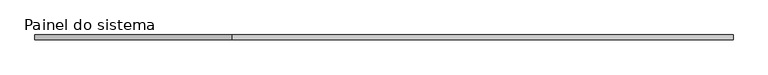
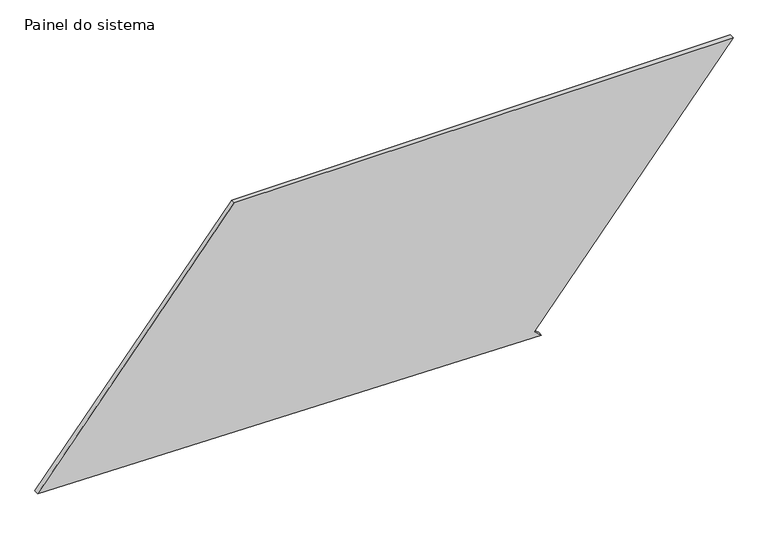
"""IFC4 building model written with IfcOpenShell, lengths in millimetres: plate geometry, Painel do sistema : Envidraçado."""

from ifc_helpers import new_model, si_unit, frame, origin, place, context, project, spatial, polyline, outline, extrude, source, transform, mapped, element, save


def painel_do_sistema_5cae5aec(model_context):
    return source(origin(), model_context, "Body", "SweptSolid", [
        extrude(outline(polyline([(0.0, 835.3915804), (31.7984882, 796.8058817), (1324.8110339, 1862.377985), (1324.8110339, -809.4089219), (47.0915773, -1862.377985), (0.0, 835.3915804)])), frame((0.0, 24.5, 0.0), z_axis=(0.0, 1.0, 0.0), x_axis=(0.0, 0.0, 1.0)), (0.0, 0.0, 1.0), 25.0),
    ])


if __name__ == "__main__":
    model = new_model("IFC4")
    model_context = context("Model", 3, world=origin())
    ifc_project = project(units=[si_unit("LENGTHUNIT", "METRE", prefix="MILLI")], contexts=[model_context])
    site = spatial("IfcSite", under=ifc_project)
    building = spatial("IfcBuilding", under=site)
    placement = place(None, origin())
    painel_do_sistema_shape = painel_do_sistema_5cae5aec(model_context)
    element("IfcPlate", 1, ObjectType="Painel do sistema : Envidraçado", at=placement, inside=building, context=model_context, shape_type="MappedRepresentation", body=[
        mapped(painel_do_sistema_shape, transform((0.0, 0.0, 0.0), x_axis=(1.0, 0.0, 0.0), y_axis=(0.0, 1.0, 0.0), z_axis=(0.0, 0.0, 1.0))),
    ])
    save(model, "model.ifc")

# Revit data of these elements
# Type "Painel do sistema : Envidraçado"
#   Construction Type Id = "GSP4R"
#   Analytic Construction = "Vidraça única Pilkington 1/8 pol"
#   Visual Light Transmittance = 0.9
#   Solar Heat Gain Coefficient = 0.86
#   Heat Transfer Coefficient (U) = 6.7069 W/(m²·K)
# Element 1 (IfcPlate, "Painel do sistema : Envidraçado")
#   Materials on its faces: "Vidro"
# Materials
#   "Vidro": class "Vidro", colour RGB 0 128 192, transparency 0.9, Description = "Vidro de sílica", Cost = 0
